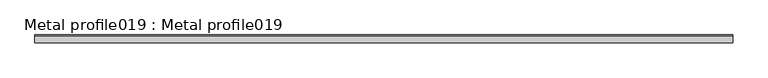
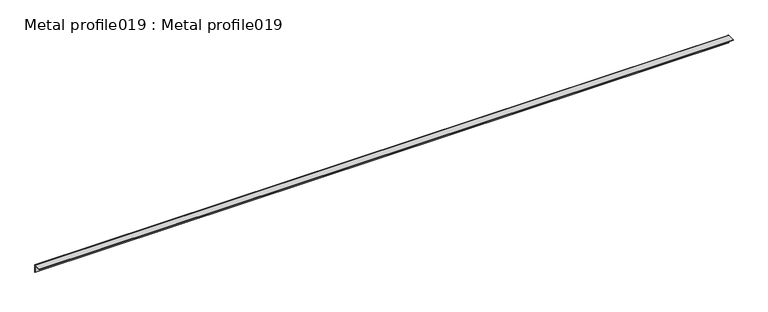
"""IFC4 building model written with IfcOpenShell, lengths in millimetres: proxy geometry, Metal profile019 : Metal profile019."""

import ifcopenshell
import ifcopenshell.guid

model = None  # the IFC model being written
_history = None  # IfcOwnerHistory: only IFC2X3 demands one
_inside = {}  # id of a spatial element -> (the spatial element, [elements in it])
_under = {}  # id of a project, library or spatial element -> (it, [spatial elements below it])
_declared = {}  # id of a project -> (the project, [libraries it declares])
_typed = {}  # id of a type object -> (the type object, [elements of that type])
_made_of = {}  # id of a material, layer set ... -> (it, [elements and type objects made of it])


def new_model(schema):
    """Start an empty IFC model of exactly this schema.

    Asked for "IFC4X3", IfcOpenShell would pick the latest addendum, in which some entities
    have other attributes; the version numbers below select the first issue.
    IFC2X3 requires an IfcOwnerHistory on every rooted entity: one is made here for all.
    """
    global model, _history
    if schema == "IFC4X3":
        model = ifcopenshell.file(schema_version=(4, 3, 0, 0))
    else:
        model = ifcopenshell.file(schema=schema)
    _inside.clear()
    _under.clear()
    _declared.clear()
    _typed.clear()
    _made_of.clear()
    _history = None
    if model.schema == "IFC2X3":
        org = make("IfcOrganization", Name="unknown")
        user = make(
            "IfcPersonAndOrganization",
            ThePerson=make("IfcPerson", FamilyName="unknown"),
            TheOrganization=org,
        )
        app = make(
            "IfcApplication",
            ApplicationDeveloper=org,
            Version="unknown",
            ApplicationFullName="unknown",
            ApplicationIdentifier="unknown",
        )
        _history = make(
            "IfcOwnerHistory",
            OwningUser=user,
            OwningApplication=app,
            ChangeAction="ADDED",
            CreationDate=0,
        )
    return model


def make(cls, **values):
    """One entity of the class cls with the attributes given. An attribute that is None is left unset."""
    return model.create_entity(
        cls, **{name: value for name, value in values.items() if value is not None}
    )


def rooted(cls, **values):
    """An entity with a GlobalId (a new one), such as an element, a storey or a relation."""
    return make(cls, GlobalId=ifcopenshell.guid.new(), OwnerHistory=_history, **values)


def si_unit(unit_type, name, prefix=None):
    """IfcSIUnit, for example si_unit("LENGTHUNIT", "METRE", prefix="MILLI")."""
    return make("IfcSIUnit", UnitType=unit_type, Prefix=prefix, Name=name)


def assignment(units):
    """IfcUnitAssignment: the units of a project."""
    return None if units is None else make("IfcUnitAssignment", Units=units)


def point(xyz):
    """IfcCartesianPoint."""
    return None if xyz is None else make("IfcCartesianPoint", Coordinates=xyz)


def direction(xyz):
    """IfcDirection."""
    return None if xyz is None else make("IfcDirection", DirectionRatios=xyz)


def frame(location, z_axis=None, x_axis=None):
    """IfcAxis2Placement3D, a coordinate frame: its origin and axes. An axis left out is left unset."""
    return make(
        "IfcAxis2Placement3D",
        Location=point(location),
        Axis=direction(z_axis),
        RefDirection=direction(x_axis),
    )


def frame_2d(location, x_axis=None):
    """IfcAxis2Placement2D, a coordinate frame in the plane: its origin and x axis."""
    return make(
        "IfcAxis2Placement2D", Location=point(location), RefDirection=direction(x_axis)
    )


def origin():
    """The frame at (0, 0, 0) with its axes left unset."""
    return frame((0.0, 0.0, 0.0))


def place(relative_to, where):
    """IfcLocalPlacement: puts the frame where relative to a parent placement (None: the world)."""
    return make(
        "IfcLocalPlacement", PlacementRelTo=relative_to, RelativePlacement=where
    )


def context(
    kind, dimensions, precision=None, world=None, true_north=None, identifier=None
):
    """IfcGeometricRepresentationContext, for example the 3D "Model" context."""
    return make(
        "IfcGeometricRepresentationContext",
        ContextIdentifier=identifier,
        ContextType=kind,
        CoordinateSpaceDimension=dimensions,
        Precision=precision,
        WorldCoordinateSystem=world,
        TrueNorth=true_north,
    )


def project(units=None, contexts=None):
    """IfcProject with its units and contexts."""
    return rooted(
        "IfcProject",
        Name="project",
        RepresentationContexts=contexts,
        UnitsInContext=assignment(units),
    )


def spatial(cls, under=None, at=None, **own):
    """A site, building, storey or space (cls), placed at a placement, below another one or the project."""
    s = rooted(cls, ObjectPlacement=at, **own)
    if under is not None:
        _under.setdefault(under.id(), (under, []))[1].append(s)
    return s


def polyline(points):
    """IfcPolyline through the points."""
    return make("IfcPolyline", Points=[point(p) for p in points])


def circle_curve(where, radius):
    """IfcCircle in the frame where."""
    return make("IfcCircle", Position=where, Radius=radius)


def trimmed(basis, trim1, trim2, sense, master):
    """IfcTrimmedCurve: the piece of a basis curve between two trims."""
    return make(
        "IfcTrimmedCurve",
        BasisCurve=basis,
        Trim1=trim1,
        Trim2=trim2,
        SenseAgreement=sense,
        MasterRepresentation=master,
    )


def segment(curve, same_sense, transition):
    """IfcCompositeCurveSegment."""
    return make(
        "IfcCompositeCurveSegment",
        Transition=transition,
        SameSense=same_sense,
        ParentCurve=curve,
    )


def composite_curve(segments, self_intersect=None):
    """IfcCompositeCurve: segments joined end to end."""
    return make("IfcCompositeCurve", Segments=segments, SelfIntersect=self_intersect)


def outline(outer, holes=None, kind="AREA"):
    """IfcArbitraryClosedProfileDef: a profile drawn as a closed curve; with holes, ...WithVoids."""
    if holes is None:
        return make("IfcArbitraryClosedProfileDef", ProfileType=kind, OuterCurve=outer)
    return make(
        "IfcArbitraryProfileDefWithVoids",
        ProfileType=kind,
        OuterCurve=outer,
        InnerCurves=holes,
    )


def extrude(swept, where, along, depth):
    """IfcExtrudedAreaSolid: the profile swept, set in the frame where, extruded along a direction by depth."""
    return make(
        "IfcExtrudedAreaSolid",
        SweptArea=swept,
        Position=where,
        ExtrudedDirection=direction(along),
        Depth=depth,
    )


def shape(context_of_items, identifier, shape_type, items):
    """IfcShapeRepresentation: the items that make up one representation, for example the "Body"."""
    return make(
        "IfcShapeRepresentation",
        ContextOfItems=context_of_items,
        RepresentationIdentifier=identifier,
        RepresentationType=shape_type,
        Items=items,
    )


def source(mapping_origin, context_of_items, identifier, shape_type, items):
    """IfcRepresentationMap: a shape defined once, which mapped items show again and again."""
    return make(
        "IfcRepresentationMap",
        MappingOrigin=mapping_origin,
        MappedRepresentation=shape(context_of_items, identifier, shape_type, items),
    )


def transform(
    local_origin,
    x_axis=None,
    y_axis=None,
    z_axis=None,
    scale=None,
    scale2=None,
    scale3=None,
    uniform=True,
):
    """IfcCartesianTransformationOperator3D, or its non-uniform kind. x_axis, y_axis, z_axis: its Axis1, 2, 3."""
    if uniform:
        return make(
            "IfcCartesianTransformationOperator3D",
            Axis1=direction(x_axis),
            Axis2=direction(y_axis),
            LocalOrigin=point(local_origin),
            Scale=scale,
            Axis3=direction(z_axis),
        )
    return make(
        "IfcCartesianTransformationOperator3DnonUniform",
        Axis1=direction(x_axis),
        Axis2=direction(y_axis),
        LocalOrigin=point(local_origin),
        Scale=scale,
        Axis3=direction(z_axis),
        Scale2=scale2,
        Scale3=scale3,
    )


def mapped(mapping_source, mapping_target):
    """IfcMappedItem: shows the shape of a source again, moved by a transform."""
    return make(
        "IfcMappedItem", MappingSource=mapping_source, MappingTarget=mapping_target
    )


def made_of(thing, what):
    """Note that an element or type object is made of a material, layer set ...; save() writes the relation."""
    if what is not None:
        _made_of.setdefault(what.id(), (what, []))[1].append(thing)
    return thing


def element(
    cls,
    number,
    at=None,
    inside=None,
    cuts=None,
    type_object=None,
    material=None,
    context=None,
    identifier="Body",
    shape_type=None,
    held_by="IfcProductDefinitionShape",
    body=None,
    shapes=None,
    **own,
):
    """One element of the class cls, such as IfcWall. Its Tag is "e" and its number.

    at: its placement. inside: the storey or other place that contains it. cuts: it is an
    opening in that element (IfcRelVoidsElement). A single representation is given by context,
    identifier, shape_type and body (its items); several are given by shapes. held_by: the class
    of the entity that holds the representations. save() writes the other relations.
    """
    e = rooted(cls, Tag="e%d" % number, ObjectPlacement=at, **own)
    if body is not None:
        shapes = [shape(context, identifier, shape_type, body)]
    if shapes is not None:
        e.Representation = make(held_by, Representations=shapes)
    if inside is not None:
        _inside.setdefault(inside.id(), (inside, []))[1].append(e)
    if cuts is not None:
        rooted(
            "IfcRelVoidsElement", RelatingBuildingElement=cuts, RelatedOpeningElement=e
        )
    if type_object is not None:
        _typed.setdefault(type_object.id(), (type_object, []))[1].append(e)
    return made_of(e, material)


def aggregate(whole, parts):
    """IfcRelAggregates: a whole, such as a stair, and the parts it consists of."""
    return rooted("IfcRelAggregates", RelatingObject=whole, RelatedObjects=parts)


def save(model, path):
    """Write the relations noted so far, then the file.

    IfcRelAggregates (storeys below a building ...), IfcRelContainedInSpatialStructure (elements
    in a storey), IfcRelDefinesByType, IfcRelAssociatesMaterial and IfcRelDeclares: one each for
    every whole, place, type object, material and project.
    """
    for whole, parts in _under.values():
        aggregate(whole, parts)
    for where, things in _inside.values():
        rooted(
            "IfcRelContainedInSpatialStructure",
            RelatedElements=things,
            RelatingStructure=where,
        )
    for kind, things in _typed.values():
        rooted("IfcRelDefinesByType", RelatedObjects=things, RelatingType=kind)
    for what, things in _made_of.values():
        rooted("IfcRelAssociatesMaterial", RelatedObjects=things, RelatingMaterial=what)
    for by, libraries in _declared.values():
        rooted("IfcRelDeclares", RelatingContext=by, RelatedDefinitions=libraries)
    model.write(path)


def metal_profile019_metal_profile019_2dac266a(model_context):
    return source(origin(), model_context, "Body", "SweptSolid", [
        extrude(outline(composite_curve([segment(polyline([(-4505.9874811, 38426.4598437), (-4505.9874811, 38427.7398437), (-4485.0845714, 38427.7398437)]), True, "CONTINUOUS"), segment(trimmed(circle_curve(frame_2d((-4484.1942972, 38427.0998437)), 1.0964434), [point((-4485.0845714, 38427.7398437))], [point((-4483.5542972, 38426.2095695))], False, "CARTESIAN"), True, "CONTINUOUS"), segment(polyline([(-4483.5542972, 38426.2095695), (-4483.5542972, 38405.3066598), (-4484.8342972, 38405.3066598), (-4484.8342972, 38426.4598437), (-4505.9874811, 38426.4598437)]), True, "CONTINUOUS")], self_intersect=False)), frame((12383.0178845, 0.0, 0.0), z_axis=(1.0, 0.0, 0.0), x_axis=(0.0, 1.0, 0.0)), (0.0, 0.0, 1.0), 2000.0),
    ])


if __name__ == "__main__":
    model = new_model("IFC4")
    model_context = context("Model", 3, world=origin())
    ifc_project = project(units=[si_unit("LENGTHUNIT", "METRE", prefix="MILLI")], contexts=[model_context])
    site = spatial("IfcSite", under=ifc_project)
    building = spatial("IfcBuilding", under=site)
    placement = place(None, origin())
    metal_profile019_metal_profile019_shape = metal_profile019_metal_profile019_2dac266a(model_context)
    element("IfcBuildingElementProxy", 1, Name="Metal profile019 : Metal profile019", ObjectType="Metal profile019 : Metal profile019", at=placement, inside=building, context=model_context, shape_type="MappedRepresentation", body=[
        mapped(metal_profile019_metal_profile019_shape, transform((0.0, 0.0, 0.0), x_axis=(1.0, 0.0, 0.0), y_axis=(0.0, 1.0, 0.0), z_axis=(0.0, 0.0, 1.0))),
    ])
    save(model, "model.ifc")

# Revit data of these elements
# Type "Metal profile019 : Metal profile019"
#   NameOverride = "Metal profile019"
# Element 1 (IfcBuildingElementProxy, "Metal profile019 : Metal profile019")
#   Materials on its faces: "CORNER BEAD"
# Materials
#   "CORNER BEAD": class "Unassigned", colour RGB 255 241 0, transparency 0
